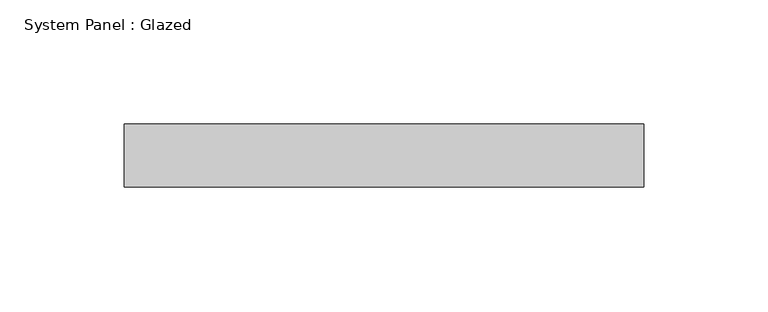
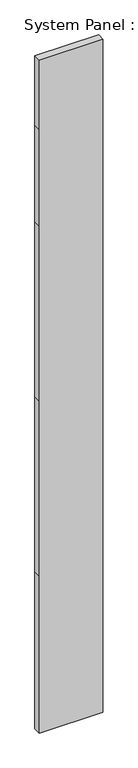
"""IFC4 building model written with IfcOpenShell, lengths in millimetres: plate geometry, System Panel : Glazed."""

from ifc_helpers import new_model, si_unit, frame, origin, place, context, project, spatial, polyline, outline, extrude, source, transform, mapped, element, save


def system_panel_glazed_9c9336f7(model_context):
    return source(origin(), model_context, "Body", "SweptSolid", [
        extrude(outline(polyline([(0.0, -104.775), (0.0, 104.775), (546.1, 104.775), (1155.7, 104.775), (1765.3, 104.775), (2101.85, 104.775), (2343.15, 104.775), (2343.15, -104.775), (2101.85, -104.775), (1765.3, -104.775), (1155.7, -104.775), (546.1, -104.775), (0.0, -104.775)])), frame((0.0, -44.45, 0.0), z_axis=(0.0, 1.0, 0.0), x_axis=(0.0, 0.0, 1.0)), (0.0, 0.0, 1.0), 25.4),
    ])


if __name__ == "__main__":
    model = new_model("IFC4")
    model_context = context("Model", 3, world=origin())
    ifc_project = project(units=[si_unit("LENGTHUNIT", "METRE", prefix="MILLI")], contexts=[model_context])
    site = spatial("IfcSite", under=ifc_project)
    building = spatial("IfcBuilding", under=site)
    placement = place(None, origin())
    system_panel_glazed_shape = system_panel_glazed_9c9336f7(model_context)
    element("IfcPlate", 1, ObjectType="System Panel : Glazed", at=placement, inside=building, context=model_context, shape_type="MappedRepresentation", body=[
        mapped(system_panel_glazed_shape, transform((0.0, 0.0, 0.0), x_axis=(1.0, 0.0, 0.0), y_axis=(0.0, 1.0, 0.0), z_axis=(0.0, 0.0, 1.0))),
    ])
    save(model, "model.ifc")

# Revit data of these elements
# Element 1 (IfcPlate, "System Panel : Glazed")
#   Materials on its faces: "Glass"
# Materials
#   "Glass": class "Glass", colour RGB 0 128 192, transparency 0.75
